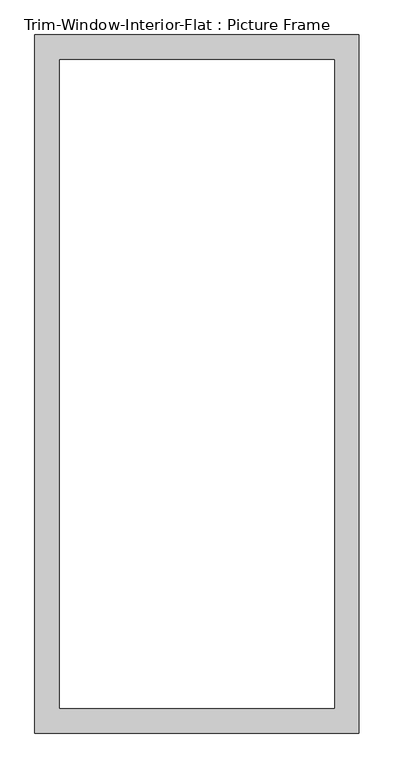
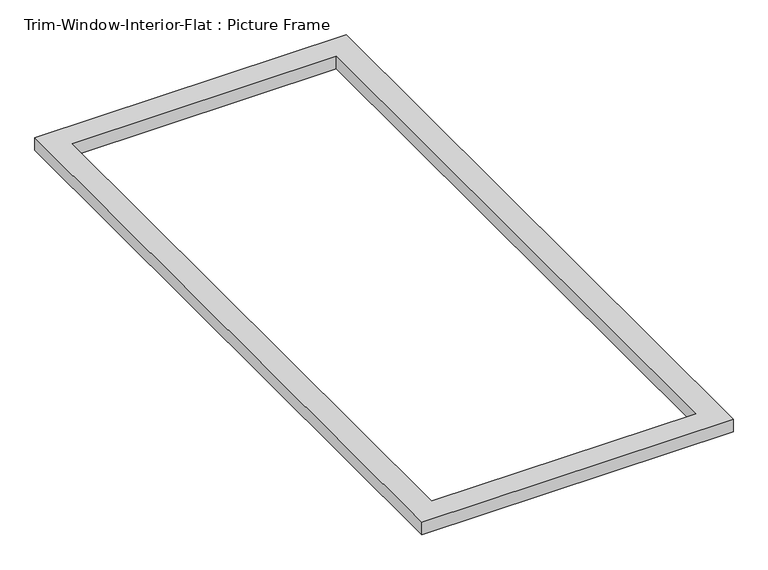
"""IFC4 building model written with IfcOpenShell, lengths in millimetres: proxy geometry, Trim-Window-Interior-Flat : Picture Frame."""

from ifc_helpers import new_model, si_unit, origin, origin_with_axes, place, context, project, spatial, polyline, outline, extrude, source, transform, mapped, element, save


def trim_window_interior_flat_picture_frame_b537ee00(model_context):
    return source(origin(), model_context, "Body", "SweptSolid", [
        extrude(outline(polyline([(374.65, -44.45), (-374.65, -44.45), (-374.65, 1568.45), (374.65, 1568.45), (374.65, -44.45)]), holes=[polyline([(317.5, 12.7), (317.5, 1511.3), (-317.5, 1511.3), (-317.5, 12.7), (317.5, 12.7)])]), origin_with_axes(), (0.0, 0.0, 1.0), 31.75),
    ])


if __name__ == "__main__":
    model = new_model("IFC4")
    model_context = context("Model", 3, world=origin())
    ifc_project = project(units=[si_unit("LENGTHUNIT", "METRE", prefix="MILLI")], contexts=[model_context])
    site = spatial("IfcSite", under=ifc_project)
    building = spatial("IfcBuilding", under=site)
    placement = place(None, origin())
    trim_window_interior_flat_picture_frame_shape = trim_window_interior_flat_picture_frame_b537ee00(model_context)
    element("IfcBuildingElementProxy", 1, Name="Trim-Window-Interior-Flat : Picture Frame", ObjectType="Trim-Window-Interior-Flat : Picture Frame", at=placement, inside=building, context=model_context, shape_type="MappedRepresentation", body=[
        mapped(trim_window_interior_flat_picture_frame_shape, transform((0.0, 0.0, 0.0), x_axis=(1.0, 0.0, 0.0), y_axis=(0.0, 1.0, 0.0), z_axis=(0.0, 0.0, 1.0))),
    ])
    save(model, "model.ifc")

# Revit data of these elements
# Type "Trim-Window-Interior-Flat : Picture Frame"
#   Trim Thickness_Picture Frame = 0' - 1 1/4"
#   Trim Width = 0' - 2 1/4"
#   Trim Thickness_with Sill = 0' - 0 3/4"
#   Sill Thickness = 0' - 1 1/4"
#   Opening Width [instance default] = 2' - 0"
#   Opening Height [instance default] = 3' - 0"
#   Default Elevation = 4' - 0"
#   Sill = no
#   Picture Frame = yes
#   Trim Material [instance default] = none
# Element 1 (IfcBuildingElementProxy, "Trim-Window-Interior-Flat : Picture Frame")
#   Opening Width = 2' - 2"
#   Opening Height = 5' - 0"
#   Trim Material = Wood - Stained
#   Materials on its faces: "Wood - Stained"
# Materials
#   "Wood - Stained": class "Wood", colour RGB 224 178 126, transparency 0, Cost = 0
